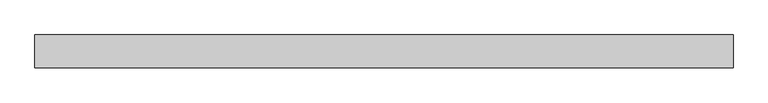
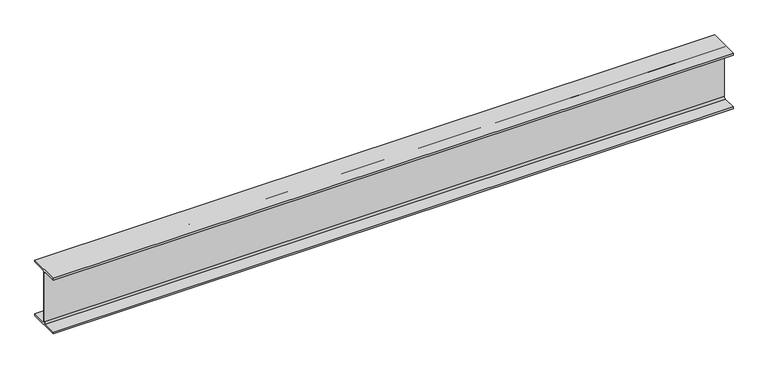
"""IFC4 building model written with IfcOpenShell, lengths in millimetres: beam geometry, Steel Beam_H-KSD3502 : H_SB_ASB_H-200x200x8x12."""

from ifc_helpers import new_model, si_unit, point, frame, frame_2d, origin, place, context, project, spatial, polyline, circle_curve, trimmed, segment, composite_curve, outline, extrude, source, transform, mapped, element, save


def beam_fe681a5f(model_context):
    return source(origin(), model_context, "Body", "SweptSolid", [
        extrude(outline(composite_curve([segment(polyline([(82.5, -141.5), (82.5, -151.7), (-82.5, -151.7), (-82.5, -141.5), (-11.9, -141.5)]), True, "CONTINUOUS"), segment(trimmed(circle_curve(frame_2d((-11.9, -132.6)), 8.9), [point((-11.9, -141.5))], [point((-3.0, -132.6))], True, "CARTESIAN"), True, "CONTINUOUS"), segment(polyline([(-3.0, -132.6), (-3.0, 132.6)]), True, "CONTINUOUS"), segment(trimmed(circle_curve(frame_2d((-11.9, 132.6)), 8.9), [point((-3.0, 132.6))], [point((-11.9, 141.5))], True, "CARTESIAN"), True, "CONTINUOUS"), segment(polyline([(-11.9, 141.5), (-82.5, 141.5), (-82.5, 151.7), (82.5, 151.7), (82.5, 141.5), (11.9, 141.5)]), True, "CONTINUOUS"), segment(trimmed(circle_curve(frame_2d((11.9, 132.6)), 8.9), [point((11.9, 141.5))], [point((3.0, 132.6))], True, "CARTESIAN"), True, "CONTINUOUS"), segment(polyline([(3.0, 132.6), (3.0, -132.6)]), True, "CONTINUOUS"), segment(trimmed(circle_curve(frame_2d((11.9, -132.6)), 8.9), [point((3.0, -132.6))], [point((11.9, -141.5))], True, "CARTESIAN"), True, "CONTINUOUS"), segment(polyline([(11.9, -141.5), (82.5, -141.5)]), True, "CONTINUOUS")], self_intersect=False)), frame((-1805.839182, 0.0, 0.0), z_axis=(1.0, 0.0, 0.0), x_axis=(0.0, 1.0, 0.0)), (0.0, 0.0, 1.0), 3511.0476207),
    ])


if __name__ == "__main__":
    model = new_model("IFC4")
    model_context = context("Model", 3, world=origin())
    ifc_project = project(units=[si_unit("LENGTHUNIT", "METRE", prefix="MILLI")], contexts=[model_context])
    site = spatial("IfcSite", under=ifc_project)
    building = spatial("IfcBuilding", under=site)
    placement = place(None, origin())
    beam_shape = beam_fe681a5f(model_context)
    element("IfcBeam", 1, ObjectType="Steel Beam_H-KSD3502 : H_SB_ASB_H-200x200x8x12", at=placement, inside=building, context=model_context, shape_type="MappedRepresentation", body=[
        mapped(beam_shape, transform((0.0, 0.0, 0.0), x_axis=(1.0, 0.0, 0.0), y_axis=(0.0, 1.0, 0.0), z_axis=(0.0, 0.0, 1.0))),
    ])
    save(model, "model.ifc")

# Revit data of these elements
# Type "Steel Beam_H-KSD3502 : H_SB_ASB_H-200x200x8x12"
#   Width = 20.0 cm
#   Web Thickness = 0.8 cm
#   Web Fillet = 1.3 cm
#   Warping Constant = 141376.0 cm⁶
#   Torsional Moment of Inertia = 26.2485 cm⁴
#   Torsional Modulus = 1.0 cm³
#   Section Area = 63.53 cm²
#   Plastic Modulus weak axis = 244.0 cm³
#   Plastic Modulus strong axis = 525.0 cm³
#   Perimeter = 1.16 m²/m
#   Nominal Weight = 49.90 kgf/m
#   Moment of Inertia weak axis = 1600.00 cm⁴
#   Moment of Inertia strong axis = 4720.00 cm⁴
#   Height = 20.0 cm
#   Flange Thickness = 1.2 cm
#   Elastic Modulus weak axis = 160.0 cm³
#   Elastic Modulus strong axis = 472.0 cm³
#   Centroid Vertical = 10.0 cm
#   Centroid Horizontal = 10.0 cm
#   Length [instance default] = 1.5240 m
#   Structural Material [instance default] = Steel, 45-345
#   Assembly Code = ""
# Element 1 (IfcBeam, "Steel Beam_H-KSD3502 : H_SB_ASB_H-200x200x8x12")
#   Structural Material = none
# Materials
#   "Steel, 45-345": class "Metal", colour RGB 189 187 185, transparency 0, Description = "Steel 345 MPa", Cost = 0
